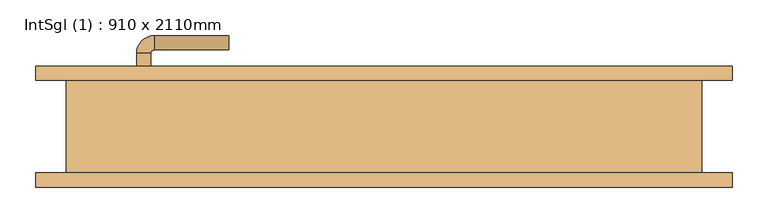
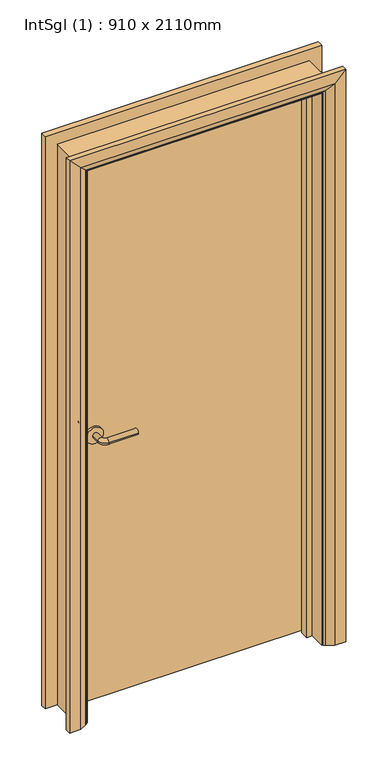
"""IFC4 building model written with IfcOpenShell, lengths in millimetres: door geometry, IntSgl (1) : 910 x 2110mm."""

import ifcopenshell
import ifcopenshell.guid

model = None  # the IFC model being written
_history = None  # IfcOwnerHistory: only IFC2X3 demands one
_inside = {}  # id of a spatial element -> (the spatial element, [elements in it])
_under = {}  # id of a project, library or spatial element -> (it, [spatial elements below it])
_declared = {}  # id of a project -> (the project, [libraries it declares])
_typed = {}  # id of a type object -> (the type object, [elements of that type])
_made_of = {}  # id of a material, layer set ... -> (it, [elements and type objects made of it])


def new_model(schema):
    """Start an empty IFC model of exactly this schema.

    Asked for "IFC4X3", IfcOpenShell would pick the latest addendum, in which some entities
    have other attributes; the version numbers below select the first issue.
    IFC2X3 requires an IfcOwnerHistory on every rooted entity: one is made here for all.
    """
    global model, _history
    if schema == "IFC4X3":
        model = ifcopenshell.file(schema_version=(4, 3, 0, 0))
    else:
        model = ifcopenshell.file(schema=schema)
    _inside.clear()
    _under.clear()
    _declared.clear()
    _typed.clear()
    _made_of.clear()
    _history = None
    if model.schema == "IFC2X3":
        org = make("IfcOrganization", Name="unknown")
        user = make(
            "IfcPersonAndOrganization",
            ThePerson=make("IfcPerson", FamilyName="unknown"),
            TheOrganization=org,
        )
        app = make(
            "IfcApplication",
            ApplicationDeveloper=org,
            Version="unknown",
            ApplicationFullName="unknown",
            ApplicationIdentifier="unknown",
        )
        _history = make(
            "IfcOwnerHistory",
            OwningUser=user,
            OwningApplication=app,
            ChangeAction="ADDED",
            CreationDate=0,
        )
    return model


def make(cls, **values):
    """One entity of the class cls with the attributes given. An attribute that is None is left unset."""
    return model.create_entity(
        cls, **{name: value for name, value in values.items() if value is not None}
    )


def rooted(cls, **values):
    """An entity with a GlobalId (a new one), such as an element, a storey or a relation."""
    return make(cls, GlobalId=ifcopenshell.guid.new(), OwnerHistory=_history, **values)


def si_unit(unit_type, name, prefix=None):
    """IfcSIUnit, for example si_unit("LENGTHUNIT", "METRE", prefix="MILLI")."""
    return make("IfcSIUnit", UnitType=unit_type, Prefix=prefix, Name=name)


def assignment(units):
    """IfcUnitAssignment: the units of a project."""
    return None if units is None else make("IfcUnitAssignment", Units=units)


def point(xyz):
    """IfcCartesianPoint."""
    return None if xyz is None else make("IfcCartesianPoint", Coordinates=xyz)


def direction(xyz):
    """IfcDirection."""
    return None if xyz is None else make("IfcDirection", DirectionRatios=xyz)


def frame(location, z_axis=None, x_axis=None):
    """IfcAxis2Placement3D, a coordinate frame: its origin and axes. An axis left out is left unset."""
    return make(
        "IfcAxis2Placement3D",
        Location=point(location),
        Axis=direction(z_axis),
        RefDirection=direction(x_axis),
    )


def frame_2d(location, x_axis=None):
    """IfcAxis2Placement2D, a coordinate frame in the plane: its origin and x axis."""
    return make(
        "IfcAxis2Placement2D", Location=point(location), RefDirection=direction(x_axis)
    )


def origin():
    """The frame at (0, 0, 0) with its axes left unset."""
    return frame((0.0, 0.0, 0.0))


def place(relative_to, where):
    """IfcLocalPlacement: puts the frame where relative to a parent placement (None: the world)."""
    return make(
        "IfcLocalPlacement", PlacementRelTo=relative_to, RelativePlacement=where
    )


def context(
    kind, dimensions, precision=None, world=None, true_north=None, identifier=None
):
    """IfcGeometricRepresentationContext, for example the 3D "Model" context."""
    return make(
        "IfcGeometricRepresentationContext",
        ContextIdentifier=identifier,
        ContextType=kind,
        CoordinateSpaceDimension=dimensions,
        Precision=precision,
        WorldCoordinateSystem=world,
        TrueNorth=true_north,
    )


def project(units=None, contexts=None):
    """IfcProject with its units and contexts."""
    return rooted(
        "IfcProject",
        Name="project",
        RepresentationContexts=contexts,
        UnitsInContext=assignment(units),
    )


def spatial(cls, under=None, at=None, **own):
    """A site, building, storey or space (cls), placed at a placement, below another one or the project."""
    s = rooted(cls, ObjectPlacement=at, **own)
    if under is not None:
        _under.setdefault(under.id(), (under, []))[1].append(s)
    return s


def polyline(points):
    """IfcPolyline through the points."""
    return make("IfcPolyline", Points=[point(p) for p in points])


def circle_curve(where, radius):
    """IfcCircle in the frame where."""
    return make("IfcCircle", Position=where, Radius=radius)


def ellipse_curve(where, semi_axis1, semi_axis2):
    """IfcEllipse in the frame where."""
    return make(
        "IfcEllipse", Position=where, SemiAxis1=semi_axis1, SemiAxis2=semi_axis2
    )


def trimmed(basis, trim1, trim2, sense, master):
    """IfcTrimmedCurve: the piece of a basis curve between two trims."""
    return make(
        "IfcTrimmedCurve",
        BasisCurve=basis,
        Trim1=trim1,
        Trim2=trim2,
        SenseAgreement=sense,
        MasterRepresentation=master,
    )


def segment(curve, same_sense, transition):
    """IfcCompositeCurveSegment."""
    return make(
        "IfcCompositeCurveSegment",
        Transition=transition,
        SameSense=same_sense,
        ParentCurve=curve,
    )


def composite_curve(segments, self_intersect=None):
    """IfcCompositeCurve: segments joined end to end."""
    return make("IfcCompositeCurve", Segments=segments, SelfIntersect=self_intersect)


def outline(outer, holes=None, kind="AREA"):
    """IfcArbitraryClosedProfileDef: a profile drawn as a closed curve; with holes, ...WithVoids."""
    if holes is None:
        return make("IfcArbitraryClosedProfileDef", ProfileType=kind, OuterCurve=outer)
    return make(
        "IfcArbitraryProfileDefWithVoids",
        ProfileType=kind,
        OuterCurve=outer,
        InnerCurves=holes,
    )


def extrude(swept, where, along, depth):
    """IfcExtrudedAreaSolid: the profile swept, set in the frame where, extruded along a direction by depth."""
    return make(
        "IfcExtrudedAreaSolid",
        SweptArea=swept,
        Position=where,
        ExtrudedDirection=direction(along),
        Depth=depth,
    )


def faces_of(points, faces, orient=None, outer=None):
    """IfcFace entities. A face is a list of loops; a loop is a list of indices into points, from 0.

    orient and outer hold one flag for each loop. By default every Orientation is true, the
    first loop of a face is its IfcFaceOuterBound and the others are IfcFaceBound.
    """
    made = []
    for i, loops in enumerate(faces):
        bounds = []
        for j, loop in enumerate(loops):
            is_outer = j == 0 if outer is None else outer[i][j]
            bounds.append(
                make(
                    "IfcFaceOuterBound" if is_outer else "IfcFaceBound",
                    Bound=make("IfcPolyLoop", Polygon=[points[k] for k in loop]),
                    Orientation=True if orient is None else orient[i][j],
                )
            )
        made.append(make("IfcFace", Bounds=bounds))
    return made


def faceted_brep(points, faces, orient=None, outer=None, voids=None):
    """IfcFacetedBrep: a solid bounded by flat faces; with voids (closed shells), ...WithVoids."""
    shared = [point(p) for p in points]
    hull = make("IfcClosedShell", CfsFaces=faces_of(shared, faces, orient, outer))
    if voids is None:
        return make("IfcFacetedBrep", Outer=hull)
    return make(
        "IfcFacetedBrepWithVoids",
        Outer=hull,
        Voids=[
            make(cls, CfsFaces=faces_of(shared, fs, o, b)) for cls, fs, o, b in voids
        ],
    )


def shape(context_of_items, identifier, shape_type, items):
    """IfcShapeRepresentation: the items that make up one representation, for example the "Body"."""
    return make(
        "IfcShapeRepresentation",
        ContextOfItems=context_of_items,
        RepresentationIdentifier=identifier,
        RepresentationType=shape_type,
        Items=items,
    )


def source(mapping_origin, context_of_items, identifier, shape_type, items):
    """IfcRepresentationMap: a shape defined once, which mapped items show again and again."""
    return make(
        "IfcRepresentationMap",
        MappingOrigin=mapping_origin,
        MappedRepresentation=shape(context_of_items, identifier, shape_type, items),
    )


def transform(
    local_origin,
    x_axis=None,
    y_axis=None,
    z_axis=None,
    scale=None,
    scale2=None,
    scale3=None,
    uniform=True,
):
    """IfcCartesianTransformationOperator3D, or its non-uniform kind. x_axis, y_axis, z_axis: its Axis1, 2, 3."""
    if uniform:
        return make(
            "IfcCartesianTransformationOperator3D",
            Axis1=direction(x_axis),
            Axis2=direction(y_axis),
            LocalOrigin=point(local_origin),
            Scale=scale,
            Axis3=direction(z_axis),
        )
    return make(
        "IfcCartesianTransformationOperator3DnonUniform",
        Axis1=direction(x_axis),
        Axis2=direction(y_axis),
        LocalOrigin=point(local_origin),
        Scale=scale,
        Axis3=direction(z_axis),
        Scale2=scale2,
        Scale3=scale3,
    )


def mapped(mapping_source, mapping_target):
    """IfcMappedItem: shows the shape of a source again, moved by a transform."""
    return make(
        "IfcMappedItem", MappingSource=mapping_source, MappingTarget=mapping_target
    )


def made_of(thing, what):
    """Note that an element or type object is made of a material, layer set ...; save() writes the relation."""
    if what is not None:
        _made_of.setdefault(what.id(), (what, []))[1].append(thing)
    return thing


def element(
    cls,
    number,
    at=None,
    inside=None,
    cuts=None,
    type_object=None,
    material=None,
    context=None,
    identifier="Body",
    shape_type=None,
    held_by="IfcProductDefinitionShape",
    body=None,
    shapes=None,
    **own,
):
    """One element of the class cls, such as IfcWall. Its Tag is "e" and its number.

    at: its placement. inside: the storey or other place that contains it. cuts: it is an
    opening in that element (IfcRelVoidsElement). A single representation is given by context,
    identifier, shape_type and body (its items); several are given by shapes. held_by: the class
    of the entity that holds the representations. save() writes the other relations.
    """
    e = rooted(cls, Tag="e%d" % number, ObjectPlacement=at, **own)
    if body is not None:
        shapes = [shape(context, identifier, shape_type, body)]
    if shapes is not None:
        e.Representation = make(held_by, Representations=shapes)
    if inside is not None:
        _inside.setdefault(inside.id(), (inside, []))[1].append(e)
    if cuts is not None:
        rooted(
            "IfcRelVoidsElement", RelatingBuildingElement=cuts, RelatedOpeningElement=e
        )
    if type_object is not None:
        _typed.setdefault(type_object.id(), (type_object, []))[1].append(e)
    return made_of(e, material)


def aggregate(whole, parts):
    """IfcRelAggregates: a whole, such as a stair, and the parts it consists of."""
    return rooted("IfcRelAggregates", RelatingObject=whole, RelatedObjects=parts)


def save(model, path):
    """Write the relations noted so far, then the file.

    IfcRelAggregates (storeys below a building ...), IfcRelContainedInSpatialStructure (elements
    in a storey), IfcRelDefinesByType, IfcRelAssociatesMaterial and IfcRelDeclares: one each for
    every whole, place, type object, material and project.
    """
    for whole, parts in _under.values():
        aggregate(whole, parts)
    for where, things in _inside.values():
        rooted(
            "IfcRelContainedInSpatialStructure",
            RelatedElements=things,
            RelatingStructure=where,
        )
    for kind, things in _typed.values():
        rooted("IfcRelDefinesByType", RelatedObjects=things, RelatingType=kind)
    for what, things in _made_of.values():
        rooted("IfcRelAssociatesMaterial", RelatedObjects=things, RelatingMaterial=what)
    for by, libraries in _declared.values():
        rooted("IfcRelDeclares", RelatingContext=by, RelatedDefinitions=libraries)
    model.write(path)


def plane_surface(at):
    """IfcPlane: the flat surface through the origin of the frame at, square to its z axis."""
    return make("IfcPlane", Position=at)


def cylinder_surface(at, radius):
    """IfcCylindricalSurface: all points at the distance radius from the z axis of the frame at."""
    return make("IfcCylindricalSurface", Position=at, Radius=radius)


def revolved_surface(curve, axis_point, axis_direction):
    """IfcSurfaceOfRevolution: the curve turned about the line through axis_point along axis_direction."""
    return make(
        "IfcSurfaceOfRevolution",
        SweptCurve=make("IfcArbitraryOpenProfileDef", ProfileType="CURVE", Curve=curve),
        AxisPosition=make("IfcAxis1Placement", Location=point(axis_point), Axis=direction(axis_direction)),
    )


def advanced_brep(points, edges, surfaces, faces):
    """IfcAdvancedBrep: a solid bounded by faces that lie on surfaces and meet in shared edges.

    An edge is (start, end): straight between two places in points (the first is 0);
    or (start, end, curve); or (start, end, curve, False) where it runs against its curve.
    A face is (place in surfaces, loops), or (place, loops, False) where it looks against
    its surface's normal. A loop lists edges by number (the first is 1), with a minus sign
    where the edge is run from its end to its start. The first loop is the outer one.
    """
    corners = [point(p) for p in points]
    vertices = [make("IfcVertexPoint", VertexGeometry=c) for c in corners]
    made = []
    for start, end, *more in edges:
        made.append(
            make(
                "IfcEdgeCurve",
                EdgeStart=vertices[start],
                EdgeEnd=vertices[end],
                EdgeGeometry=more[0] if more else make("IfcPolyline", Points=[corners[start], corners[end]]),
                SameSense=more[1] if len(more) > 1 else True,
            )
        )
    hull = []
    for where, loops, *sense in faces:
        bounds = []
        for j, loop in enumerate(loops):
            ring = [make("IfcOrientedEdge", EdgeElement=made[abs(k) - 1], Orientation=k > 0) for k in loop]
            bounds.append(
                make(
                    "IfcFaceOuterBound" if j == 0 else "IfcFaceBound",
                    Bound=make("IfcEdgeLoop", EdgeList=ring),
                    Orientation=True,
                )
            )
        hull.append(make("IfcAdvancedFace", Bounds=bounds, FaceSurface=surfaces[where], SameSense=sense[0] if sense else True))
    return make("IfcAdvancedBrep", Outer=make("IfcClosedShell", CfsFaces=hull))


def intsgl_1_910_x_2110mm_3ac1de32(model_context):
    return source(origin(), model_context, "Body", "SolidModel", [
        advanced_brep(
        [(-348.0, 19.0, 1000.0), (-328.0, 19.0, 1000.0), (-328.0, -11.0, 1000.0), (-348.0, -11.0, 1000.0), (-323.0, -16.0, 1000.0), (-323.0, -36.0, 1000.0), (-218.0, -36.0, 1000.0), (-218.0, -16.0, 1000.0)],
        [
            (0, 1, circle_curve(frame((-338.0, 19.0, 1000.0), z_axis=(0.0, 1.0, 0.0), x_axis=(1.0, 0.0, 0.0)), 10.0)),
            (1, 0, circle_curve(frame((-338.0, 19.0, 1000.0), z_axis=(0.0, 1.0, 0.0), x_axis=(1.0, 0.0, 0.0)), 10.0)),
            (1, 2),
            (2, 3, circle_curve(frame((-338.0, -11.0, 1000.0), z_axis=(0.0, 1.0, 0.0), x_axis=(1.0, 0.0, 0.0)), 10.0)),
            (3, 0),
            (3, 2, circle_curve(frame((-338.0, -11.0, 1000.0), z_axis=(0.0, 1.0, 0.0), x_axis=(1.0, 0.0, 0.0)), 10.0)),
            (4, 5, circle_curve(frame((-323.0, -26.0, 1000.0), z_axis=(-1.0, 0.0, 0.0), x_axis=(0.0, 1.0, 0.0)), 10.0)),
            (5, 3, circle_curve(frame((-323.0, -11.0, 1000.0), z_axis=(0.0, 0.0, -1.0), x_axis=(-1.0, 0.0, 0.0)), 25.0)),
            (2, 4, circle_curve(frame((-323.0, -11.0, 1000.0), z_axis=(0.0, 0.0, 1.0), x_axis=(-1.0, 0.0, 0.0)), 5.0)),
            (5, 4, circle_curve(frame((-323.0, -26.0, 1000.0), z_axis=(-1.0, 0.0, 0.0), x_axis=(0.0, 1.0, 0.0)), 10.0)),
            (6, 7, circle_curve(frame((-218.0, -26.0, 1000.0), z_axis=(1.0, 0.0, 0.0), x_axis=(0.0, 1.0, 0.0)), 10.0)),
            (7, 6, circle_curve(frame((-218.0, -26.0, 1000.0), z_axis=(1.0, 0.0, 0.0), x_axis=(0.0, 1.0, 0.0)), 10.0)),
            (4, 7),
            (6, 5),
        ],
        [
            plane_surface(frame((-338.0, 19.0, 1000.0), z_axis=(0.0, 1.0, 0.0), x_axis=(0.0, 0.0, 1.0))),
            cylinder_surface(frame((-338.0, 19.0, 1000.0), z_axis=(0.0, 1.0, 0.0), x_axis=(1.0, 0.0, 0.0)), 10.0),
            revolved_surface(trimmed(ellipse_curve(frame((-338.0, -11.0, 1000.0), z_axis=(0.0, -1.0, 0.0), x_axis=(1.0, 0.0, 0.0)), 10.0, 10.0), [point((-348.0, -11.0, 1000.0))], [point((-328.0, -11.0, 1000.0))], True, "CARTESIAN"), (-323.0, -11.0, 1000.0), (0.0, 0.0, -1.0)),
            revolved_surface(trimmed(ellipse_curve(frame((-338.0, -11.0, 1000.0), z_axis=(0.0, -1.0, 0.0), x_axis=(1.0, 0.0, 0.0)), 10.0, 10.0), [point((-328.0, -11.0, 1000.0))], [point((-348.0, -11.0, 1000.0))], True, "CARTESIAN"), (-323.0, -11.0, 1000.0), (0.0, 0.0, -1.0)),
            plane_surface(frame((-218.0, -26.0, 1000.0), z_axis=(1.0, 0.0, 0.0), x_axis=(0.0, 0.0, 1.0))),
            cylinder_surface(frame((-323.0, -26.0, 1000.0), z_axis=(-1.0, 0.0, 0.0), x_axis=(0.0, 1.0, 0.0)), 10.0),
        ],
        [
            (0, [[1, 2]]),
            (1, [[3, 4, 5, -2]]),
            (1, [[-5, 6, -3, -1]]),
            (2, [[7, 8, -4, 9]]),
            (3, [[10, -9, -6, -8]]),
            (4, [[11, 12]]),
            (5, [[13, -11, 14, -7]]),
            (5, [[-14, -12, -13, -10]]),
        ],
    ),
        extrude(outline(composite_curve([segment(trimmed(circle_curve(frame_2d((1000.0, -340.5)), 30.0), [point((1000.0, -370.5))], [point((1000.0, -310.5))], False, "CARTESIAN"), True, "CONTINUOUS"), segment(trimmed(circle_curve(frame_2d((1000.0, -340.5)), 30.0), [point((1000.0, -310.5))], [point((1000.0, -370.5))], False, "CARTESIAN"), True, "CONTINUOUS")], self_intersect=False)), frame((0.0, 19.0, 0.0), z_axis=(0.0, 1.0, 0.0), x_axis=(0.0, 0.0, 1.0)), (0.0, 0.0, 1.0), 8.0),
        advanced_brep(
        [(-348.0, 73.0, 1000.0), (-328.0, 73.0, 1000.0), (-348.0, 103.0, 1000.0), (-328.0, 103.0, 1000.0), (-323.0, 108.0, 1000.0), (-323.0, 128.0, 1000.0), (-218.0, 128.0, 1000.0), (-218.0, 108.0, 1000.0)],
        [
            (0, 1, circle_curve(frame((-338.0, 73.0, 1000.0), z_axis=(0.0, -1.0, 0.0), x_axis=(1.0, 0.0, 0.0)), 10.0)),
            (1, 0, circle_curve(frame((-338.0, 73.0, 1000.0), z_axis=(0.0, -1.0, 0.0), x_axis=(1.0, 0.0, 0.0)), 10.0)),
            (0, 2),
            (2, 3, circle_curve(frame((-338.0, 103.0, 1000.0), z_axis=(0.0, -1.0, 0.0), x_axis=(1.0, 0.0, 0.0)), 10.0)),
            (3, 1),
            (3, 2, circle_curve(frame((-338.0, 103.0, 1000.0), z_axis=(0.0, -1.0, 0.0), x_axis=(1.0, 0.0, 0.0)), 10.0)),
            (4, 3, circle_curve(frame((-323.0, 103.0, 1000.0), z_axis=(0.0, 0.0, 1.0), x_axis=(-1.0, 0.0, 0.0)), 5.0)),
            (2, 5, circle_curve(frame((-323.0, 103.0, 1000.0), z_axis=(0.0, 0.0, -1.0), x_axis=(-1.0, 0.0, 0.0)), 25.0)),
            (5, 4, circle_curve(frame((-323.0, 118.0, 1000.0), z_axis=(-1.0, 0.0, 0.0), x_axis=(0.0, -1.0, 0.0)), 10.0)),
            (4, 5, circle_curve(frame((-323.0, 118.0, 1000.0), z_axis=(-1.0, 0.0, 0.0), x_axis=(0.0, -1.0, 0.0)), 10.0)),
            (6, 7, circle_curve(frame((-218.0, 118.0, 1000.0), z_axis=(1.0, 0.0, 0.0), x_axis=(0.0, -1.0, 0.0)), 10.0)),
            (7, 6, circle_curve(frame((-218.0, 118.0, 1000.0), z_axis=(1.0, 0.0, 0.0), x_axis=(0.0, -1.0, 0.0)), 10.0)),
            (5, 6),
            (7, 4),
        ],
        [
            plane_surface(frame((-338.0, 73.0, 1000.0), z_axis=(0.0, -1.0, 0.0), x_axis=(0.0, 0.0, 1.0))),
            cylinder_surface(frame((-338.0, 73.0, 1000.0), z_axis=(0.0, -1.0, 0.0), x_axis=(1.0, 0.0, 0.0)), 10.0),
            revolved_surface(trimmed(ellipse_curve(frame((-338.0, 103.0, 1000.0), z_axis=(0.0, -1.0, 0.0), x_axis=(1.0, 0.0, 0.0)), 10.0, 10.0), [point((-348.0, 103.0, 1000.0))], [point((-328.0, 103.0, 1000.0))], True, "CARTESIAN"), (-323.0, 103.0, 1000.0), (0.0, 0.0, -1.0)),
            revolved_surface(trimmed(ellipse_curve(frame((-338.0, 103.0, 1000.0), z_axis=(0.0, -1.0, 0.0), x_axis=(1.0, 0.0, 0.0)), 10.0, 10.0), [point((-328.0, 103.0, 1000.0))], [point((-348.0, 103.0, 1000.0))], True, "CARTESIAN"), (-323.0, 103.0, 1000.0), (0.0, 0.0, -1.0)),
            plane_surface(frame((-218.0, 118.0, 1000.0), z_axis=(1.0, 0.0, 0.0), x_axis=(0.0, 0.0, 1.0))),
            cylinder_surface(frame((-323.0, 118.0, 1000.0), z_axis=(-1.0, 0.0, 0.0), x_axis=(0.0, -1.0, 0.0)), 10.0),
        ],
        [
            (0, [[1, 2]]),
            (1, [[-1, 3, 4, 5]]),
            (1, [[-2, -5, 6, -3]]),
            (2, [[7, -4, 8, 9]]),
            (3, [[-8, -6, -7, 10]]),
            (4, [[11, 12]]),
            (5, [[-9, 13, -12, 14]]),
            (5, [[-10, -14, -11, -13]]),
        ],
    ),
        extrude(outline(composite_curve([segment(trimmed(circle_curve(frame_2d((1000.0, -340.5)), 30.0), [point((1000.0, -370.5))], [point((1000.0, -310.5))], False, "CARTESIAN"), True, "CONTINUOUS"), segment(trimmed(circle_curve(frame_2d((1000.0, -340.5)), 30.0), [point((1000.0, -310.5))], [point((1000.0, -370.5))], False, "CARTESIAN"), True, "CONTINUOUS")], self_intersect=False)), frame((0.0, 65.0, 0.0), z_axis=(0.0, 1.0, 0.0), x_axis=(0.0, 0.0, 1.0)), (0.0, 0.0, 1.0), 8.0),
        extrude(outline(polyline([(413.0, 27.0), (-413.0, 27.0), (-413.0, 65.0), (413.0, 65.0), (413.0, 27.0)])), frame((0.0, 0.0, 8.0), z_axis=(0.0, 0.0, 1.0), x_axis=(1.0, 0.0, 0.0)), (0.0, 0.0, 1.0), 2060.0),
        advanced_brep(
        [(490.0, 85.0, 0.0), (490.0, 65.0, 0.0), (420.0, 65.0, 0.0), (424.0, 71.0, 0.0), (450.0, 85.0, 0.0), (490.0, 85.0, 2145.0), (490.0, 65.0, 2145.0), (-490.0, 65.0, 2145.0), (-490.0, 65.0, 0.0), (-420.0, 65.0, 0.0), (-420.0, 65.0, 2075.0), (420.0, 65.0, 2075.0), (424.0, 71.0, 2079.0), (450.0, 85.0, 2105.0), (-450.0, 85.0, 2105.0), (-450.0, 85.0, 0.0), (-490.0, 85.0, 0.0), (-490.0, 85.0, 2145.0), (-424.0, 71.0, 2079.0), (-424.0, 71.0, 0.0)],
        [
            (0, 1),
            (1, 2),
            (2, 3, circle_curve(frame((428.0, 64.0, 0.0), z_axis=(0.0, 0.0, -1.0), x_axis=(1.0, 0.0, 0.0)), 8.0622577)),
            (3, 4),
            (4, 0),
            (0, 5),
            (5, 6),
            (6, 1),
            (6, 7),
            (7, 8),
            (8, 9),
            (9, 10),
            (10, 11),
            (11, 2),
            (11, 12, ellipse_curve(frame((428.0, 64.0, 2083.0), z_axis=(0.7071067811865475, 0.0, -0.7071067811865475), x_axis=(-0.7071067811865474, 0.0, -0.7071067811865476)), 11.4017543, 8.0622577)),
            (12, 3),
            (12, 13),
            (13, 4),
            (13, 14),
            (14, 15),
            (15, 16),
            (16, 17),
            (17, 5),
            (17, 7),
            (10, 18, ellipse_curve(frame((-428.0, 64.0, 2083.0), z_axis=(0.7071067811865475, 0.0, 0.7071067811865475), x_axis=(0.7071067811865476, 0.0, -0.7071067811865474)), 11.4017543, 8.0622577)),
            (18, 12),
            (18, 14),
            (15, 19),
            (19, 9, circle_curve(frame((-428.0, 64.0, 0.0), z_axis=(0.0, 0.0, -1.0), x_axis=(-1.0, 0.0, 0.0)), 8.0622577)),
            (8, 16),
            (19, 18),
        ],
        [
            plane_surface(frame((420.0, 65.0, 0.0), z_axis=(0.0, 0.0, -1.0), x_axis=(0.0, -1.0, 0.0))),
            plane_surface(frame((490.0, 85.0, 0.0), z_axis=(1.0, 0.0, 0.0), x_axis=(0.0, 0.0, 1.0))),
            plane_surface(frame((490.0, 65.0, 0.0), z_axis=(0.0, -1.0, 0.0), x_axis=(0.0, 0.0, 1.0))),
            cylinder_surface(frame((428.0, 64.0, 0.0), z_axis=(0.0, 0.0, -1.0), x_axis=(1.0, 0.0, 0.0)), 8.0622577),
            plane_surface(frame((424.0, 71.0, 0.0), z_axis=(-0.4740998230350126, 0.880471099922178, 0.0), x_axis=(0.0, 0.0, 1.0))),
            plane_surface(frame((450.0, 85.0, 0.0), z_axis=(0.0, 1.0, 0.0), x_axis=(0.0, 0.0, 1.0))),
            plane_surface(frame((490.0, 85.0, 2145.0), z_axis=(0.0, 0.0, 1.0), x_axis=(-1.0, 0.0, 0.0))),
            cylinder_surface(frame((420.0, 64.0, 2083.0), z_axis=(1.0, 0.0, 0.0), x_axis=(0.0, 0.0, 1.0)), 8.0622577),
            plane_surface(frame((424.0, 71.0, 2079.0), z_axis=(0.0, 0.8804710999221764, -0.4740998230350154), x_axis=(-1.0, 0.0, 0.0))),
            plane_surface(frame((-420.0, 65.0, 0.0), z_axis=(0.0, 0.0, -1.0), x_axis=(0.0, -1.0, 0.0))),
            plane_surface(frame((-490.0, 85.0, 2145.0), z_axis=(-1.0, 0.0, 0.0), x_axis=(0.0, 0.0, -1.0))),
            cylinder_surface(frame((-428.0, 64.0, 2075.0), z_axis=(0.0, 0.0, 1.0), x_axis=(-1.0, 0.0, 0.0)), 8.0622577),
            plane_surface(frame((-424.0, 71.0, 2079.0), z_axis=(0.47409982303501824, 0.8804710999221749, 0.0), x_axis=(0.0, 0.0, -1.0))),
        ],
        [
            (0, [[1, 2, 3, 4, 5]]),
            (1, [[-1, 6, 7, 8]]),
            (2, [[-2, -8, 9, 10, 11, 12, 13, 14]]),
            (3, [[-3, -14, 15, 16]]),
            (4, [[-4, -16, 17, 18]]),
            (5, [[-5, -18, 19, 20, 21, 22, 23, -6]]),
            (6, [[-7, -23, 24, -9]]),
            (7, [[-15, -13, 25, 26]]),
            (8, [[-17, -26, 27, -19]]),
            (9, [[-21, 28, 29, -11, 30]]),
            (10, [[-24, -22, -30, -10]]),
            (11, [[-25, -12, -29, 31]]),
            (12, [[-27, -31, -28, -20]]),
        ],
    ),
        extrude(outline(polyline([(0.0, -415.0), (0.0, -396.0), (2051.0, -396.0), (2051.0, 396.0), (0.0, 396.0), (0.0, 415.0), (2070.0, 415.0), (2070.0, -415.0), (0.0, -415.0)])), frame((0.0, -7.0, 0.0), z_axis=(0.0, 1.0, 0.0), x_axis=(0.0, 0.0, 1.0)), (0.0, 0.0, 1.0), 32.0),
        advanced_brep(
        [(-490.0, -85.0, 0.0), (-490.0, -65.0, 0.0), (-420.0, -65.0, 0.0), (-424.0, -71.0, 0.0), (-450.0, -85.0, 0.0), (-490.0, -85.0, 2145.0), (-490.0, -65.0, 2145.0), (-420.0, -65.0, 2075.0), (-424.0, -71.0, 2079.0), (-450.0, -85.0, 2105.0), (490.0, -85.0, 2145.0), (490.0, -65.0, 2145.0), (420.0, -65.0, 2075.0), (424.0, -71.0, 2079.0), (450.0, -85.0, 2105.0), (490.0, -85.0, 0.0), (450.0, -85.0, 0.0), (424.0, -71.0, 0.0), (420.0, -65.0, 0.0), (490.0, -65.0, 0.0)],
        [
            (0, 1),
            (1, 2),
            (2, 3, circle_curve(frame((-428.0, -64.0, 0.0), z_axis=(0.0, 0.0, -1.0), x_axis=(-1.0, 0.0, 0.0)), 8.0622577)),
            (3, 4),
            (4, 0),
            (0, 5),
            (5, 6),
            (6, 1),
            (6, 7),
            (7, 2),
            (7, 8, ellipse_curve(frame((-428.0, -64.0, 2083.0), z_axis=(-0.7071067811865475, 0.0, -0.7071067811865475), x_axis=(0.7071067811865474, 0.0, -0.7071067811865476)), 11.4017543, 8.0622577)),
            (8, 3),
            (8, 9),
            (9, 4),
            (9, 5),
            (5, 10),
            (10, 11),
            (11, 6),
            (11, 12),
            (12, 7),
            (12, 13, ellipse_curve(frame((428.0, -64.0, 2083.0), z_axis=(-0.7071067811865475, 0.0, 0.7071067811865475), x_axis=(-0.7071067811865476, 0.0, -0.7071067811865474)), 11.4017543, 8.0622577)),
            (13, 8),
            (13, 14),
            (14, 9),
            (14, 10),
            (15, 16),
            (16, 17),
            (17, 18, circle_curve(frame((428.0, -64.0, 0.0), z_axis=(0.0, 0.0, -1.0), x_axis=(1.0, 0.0, 0.0)), 8.0622577)),
            (18, 19),
            (19, 15),
            (10, 15),
            (19, 11),
            (18, 12),
            (17, 13),
            (16, 14),
        ],
        [
            plane_surface(frame((-420.0, -137.8010989, 0.0), z_axis=(0.0, 0.0, -1.0), x_axis=(1.0, 0.0, 0.0))),
            plane_surface(frame((-490.0, -85.0, 0.0), z_axis=(-1.0, 0.0, 0.0), x_axis=(0.0, 0.0, 1.0))),
            plane_surface(frame((-490.0, -65.0, 0.0), z_axis=(0.0, 1.0, 0.0), x_axis=(0.0, 0.0, 1.0))),
            cylinder_surface(frame((-428.0, -64.0, 0.0), z_axis=(0.0, 0.0, -1.0), x_axis=(-1.0, 0.0, 0.0)), 8.0622577),
            plane_surface(frame((-424.0, -71.0, 0.0), z_axis=(0.4740998230350183, -0.8804710999221749, 0.0), x_axis=(0.0, 0.0, 1.0))),
            plane_surface(frame((-450.0, -85.0, 0.0), z_axis=(0.0, -1.0, 0.0), x_axis=(0.0, 0.0, 1.0))),
            plane_surface(frame((-490.0, -85.0, 2145.0), z_axis=(0.0, 0.0, 1.0), x_axis=(1.0, 0.0, 0.0))),
            plane_surface(frame((-490.0, -65.0, 2145.0), z_axis=(0.0, 1.0, 0.0), x_axis=(1.0, 0.0, 0.0))),
            cylinder_surface(frame((-420.0, -64.0, 2083.0), z_axis=(-1.0, 0.0, 0.0), x_axis=(0.0, 0.0, 1.0)), 8.0622577),
            plane_surface(frame((-424.0, -71.0, 2079.0), z_axis=(0.0, -0.8804710999221749, -0.4740998230350183), x_axis=(1.0, 0.0, 0.0))),
            plane_surface(frame((-450.0, -85.0, 2105.0), z_axis=(0.0, -1.0, 0.0), x_axis=(1.0, 0.0, 0.0))),
            plane_surface(frame((420.0, -137.8010989, 0.0), z_axis=(0.0, 0.0, -1.0), x_axis=(-1.0, 0.0, 0.0))),
            plane_surface(frame((490.0, -85.0, 2145.0), z_axis=(1.0, 0.0, 0.0), x_axis=(0.0, 0.0, -1.0))),
            plane_surface(frame((490.0, -65.0, 2145.0), z_axis=(0.0, 1.0, 0.0), x_axis=(0.0, 0.0, -1.0))),
            cylinder_surface(frame((428.0, -64.0, 2075.0), z_axis=(0.0, 0.0, 1.0), x_axis=(1.0, 0.0, 0.0)), 8.0622577),
            plane_surface(frame((424.0, -71.0, 2079.0), z_axis=(-0.4740998230350183, -0.8804710999221749, 0.0), x_axis=(0.0, 0.0, -1.0))),
            plane_surface(frame((450.0, -85.0, 2105.0), z_axis=(0.0, -1.0, 0.0), x_axis=(0.0, 0.0, -1.0))),
        ],
        [
            (0, [[1, 2, 3, 4, 5]]),
            (1, [[-1, 6, 7, 8]]),
            (2, [[-2, -8, 9, 10]]),
            (3, [[-3, -10, 11, 12]]),
            (4, [[-4, -12, 13, 14]]),
            (5, [[-5, -14, 15, -6]]),
            (6, [[-7, 16, 17, 18]]),
            (7, [[-9, -18, 19, 20]]),
            (8, [[-11, -20, 21, 22]]),
            (9, [[-13, -22, 23, 24]]),
            (10, [[-15, -24, 25, -16]]),
            (11, [[26, 27, 28, 29, 30]]),
            (12, [[-17, 31, -30, 32]]),
            (13, [[-19, -32, -29, 33]]),
            (14, [[-21, -33, -28, 34]]),
            (15, [[-23, -34, -27, 35]]),
            (16, [[-25, -35, -26, -31]]),
        ],
    ),
        faceted_brep([(-415.0, 65.0, 0.0), (-415.0, -65.0, 0.0), (-447.0, -65.0, 0.0), (-447.0, 65.0, 0.0), (-415.0, 65.0, 2070.0), (-415.0, -65.0, 2070.0), (-447.0, -65.0, 2102.0), (-447.0, 65.0, 2102.0), (415.0, 65.0, 2070.0), (415.0, -65.0, 2070.0), (447.0, -65.0, 2102.0), (447.0, 65.0, 2102.0), (415.0, 65.0, 0.0), (447.0, 65.0, 0.0), (447.0, -65.0, 0.0), (415.0, -65.0, 0.0)], [[[0, 1, 2, 3]], [[1, 0, 4, 5]], [[2, 1, 5, 6]], [[3, 2, 6, 7]], [[0, 3, 7, 4]], [[5, 4, 8, 9]], [[6, 5, 9, 10]], [[7, 6, 10, 11]], [[4, 7, 11, 8]], [[12, 13, 14, 15]], [[9, 8, 12, 15]], [[10, 9, 15, 14]], [[11, 10, 14, 13]], [[8, 11, 13, 12]]]),
    ])


if __name__ == "__main__":
    model = new_model("IFC4")
    model_context = context("Model", 3, world=origin())
    ifc_project = project(units=[si_unit("LENGTHUNIT", "METRE", prefix="MILLI")], contexts=[model_context])
    site = spatial("IfcSite", under=ifc_project)
    building = spatial("IfcBuilding", under=site)
    placement = place(None, origin())
    intsgl_1_910_x_2110mm_shape = intsgl_1_910_x_2110mm_3ac1de32(model_context)
    element("IfcDoor", 1, ObjectType="IntSgl (1) : 910 x 2110mm", at=placement, inside=building, context=model_context, shape_type="MappedRepresentation", body=[
        mapped(intsgl_1_910_x_2110mm_shape, transform((0.0, 0.0, 0.0), x_axis=(1.0, 0.0, 0.0), y_axis=(0.0, 1.0, 0.0), z_axis=(0.0, 0.0, 1.0))),
    ])
    save(model, "model.ifc")

# Revit data of these elements
# Type "IntSgl (1) : 910 x 2110mm"
#   Construction Type Id = "MDOOR"
#   Analytic Construction = "Metal"
#   Type Mark = "41"
#   Type Comments = "Internal Single"
#   Operation = "SingleSwingRight"
#   Manufacturer = "Revit"
#   Keynote = "L20"
#   Description = "Internal Single Door"
#   Visual Light Transmittance = 0
#   Solar Heat Gain Coefficient = 0
#   Heat Transfer Coefficient (U) = 3.7021 W/(m²·K)
#   UnderCut = 8 mm
#   Tolerance = 2 mm
#   Thickness = 38 mm
#   Structural Tolerance = 8 mm
#   StopDepth = 32 mm
#   Stop Thickness = 19 mm
#   Rough Width = 910 mm
#   Rough Height = 2110 mm
#   Height to Top Lock Rail = 1000 mm
#   Handle Z Distance = 1000 mm
#   Handle X Distance = 75 mm
#   Frame Thickness = 32 mm
#   Door Panel Width = 826 mm
#   Door Panel Thickness = 38 mm
#   Door Panel Offset = 0 mm
#   Height = 2110 mm
#   Width = 910 mm
#   Door Panel Height = 2060 mm
#   Architrave Setback = 5 mm
#   Function = 0
#   Vis - Ironmongery = yes
#   Material Ironmongery = Door - Handle
#   Material Frame = Door - Frame/Mullion (1)
#   Material Door = Door - Panel
#   Material Architrave = Door - Architrave
#   Wall Closure = (empty or 0)
# Element 1 (IfcDoor, "IntSgl (1) : 910 x 2110mm")
#   Materials on its faces: "Door - Architrave", "Door - Handle", "Door - Frame/Mullion (1)", "Door - Panel"
# Materials
#   "Door - Handle": class "Miscellaneous", colour RGB 0 0 0, transparency 0, Keynote = "P21"
#   "Door - Frame/Mullion (1)": class "Wood", colour RGB 212 179 113, transparency 0, Keynote = "L20", Cost = 0
#   "Door - Panel": class "Wood", colour RGB 210 159 95, transparency 0, Keynote = "L20"
#   "Door - Architrave": class "Wood", colour RGB 154 90 5, transparency 0, Keynote = "P20"
